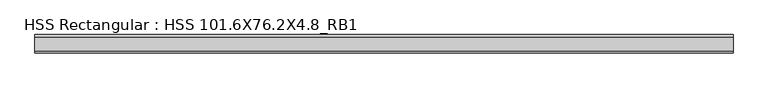
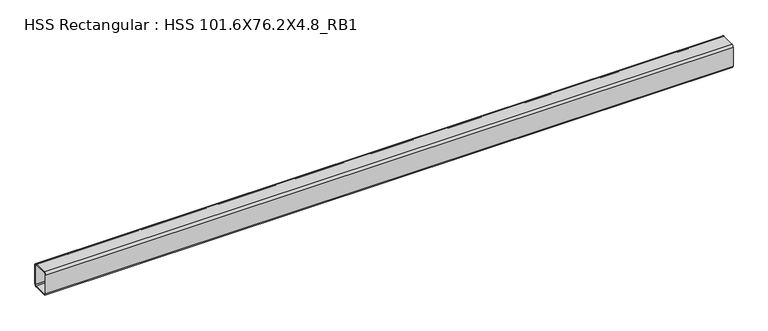
"""IFC4 building model written with IfcOpenShell, lengths in millimetres: beam geometry, HSS Rectangular : HSS 101.6X76.2X4.8_RB1."""

from ifc_helpers import new_model, si_unit, point, frame, frame_2d, origin, place, context, project, spatial, polyline, circle_curve, trimmed, segment, composite_curve, outline, extrude, source, transform, mapped, element, save


def hss_rectangular_hss_101_6x76_2x4_8_rb1_4e28bed8(model_context):
    return source(origin(), model_context, "Body", "SweptSolid", [
        extrude(outline(composite_curve([segment(polyline([(38.1, 41.275), (38.1, -41.275)]), True, "CONTINUOUS"), segment(trimmed(circle_curve(frame_2d((28.575, -41.275)), 9.525), [point((38.1, -41.275))], [point((28.575, -50.8))], False, "CARTESIAN"), True, "CONTINUOUS"), segment(polyline([(28.575, -50.8), (-28.575, -50.8)]), True, "CONTINUOUS"), segment(trimmed(circle_curve(frame_2d((-28.575, -41.275)), 9.525), [point((-28.575, -50.8))], [point((-38.1, -41.275))], False, "CARTESIAN"), True, "CONTINUOUS"), segment(polyline([(-38.1, -41.275), (-38.1, 41.275)]), True, "CONTINUOUS"), segment(trimmed(circle_curve(frame_2d((-28.575, 41.275)), 9.525), [point((-38.1, 41.275))], [point((-28.575, 50.8))], False, "CARTESIAN"), True, "CONTINUOUS"), segment(polyline([(-28.575, 50.8), (28.575, 50.8)]), True, "CONTINUOUS"), segment(trimmed(circle_curve(frame_2d((28.575, 41.275)), 9.525), [point((28.575, 50.8))], [point((38.1, 41.275))], False, "CARTESIAN"), True, "CONTINUOUS")], self_intersect=False), holes=[composite_curve([segment(trimmed(circle_curve(frame_2d((-28.575, 41.275)), 4.7625), [point((-28.575, 46.0375))], [point((-33.3375, 41.275))], True, "CARTESIAN"), True, "CONTINUOUS"), segment(polyline([(-33.3375, 41.275), (-33.3375, -41.275)]), True, "CONTINUOUS"), segment(trimmed(circle_curve(frame_2d((-28.575, -41.275)), 4.7625), [point((-33.3375, -41.275))], [point((-28.575, -46.0375))], True, "CARTESIAN"), True, "CONTINUOUS"), segment(polyline([(-28.575, -46.0375), (28.575, -46.0375)]), True, "CONTINUOUS"), segment(trimmed(circle_curve(frame_2d((28.575, -41.275)), 4.7625), [point((28.575, -46.0375))], [point((33.3375, -41.275))], True, "CARTESIAN"), True, "CONTINUOUS"), segment(polyline([(33.3375, -41.275), (33.3375, 41.275)]), True, "CONTINUOUS"), segment(trimmed(circle_curve(frame_2d((28.575, 41.275)), 4.7625), [point((33.3375, 41.275))], [point((28.575, 46.0375))], True, "CARTESIAN"), True, "CONTINUOUS"), segment(polyline([(28.575, 46.0375), (-28.575, 46.0375)]), True, "CONTINUOUS")], self_intersect=False)]), frame((-1474.1250006, 0.0, 0.0), z_axis=(1.0, 0.0, 0.0), x_axis=(0.0, 1.0, 0.0)), (0.0, 0.0, 1.0), 2884.7500012),
    ])


if __name__ == "__main__":
    model = new_model("IFC4")
    model_context = context("Model", 3, world=origin())
    ifc_project = project(units=[si_unit("LENGTHUNIT", "METRE", prefix="MILLI")], contexts=[model_context])
    site = spatial("IfcSite", under=ifc_project)
    building = spatial("IfcBuilding", under=site)
    placement = place(None, origin())
    hss_rectangular_hss_101_6x76_2x4_8_rb1_shape = hss_rectangular_hss_101_6x76_2x4_8_rb1_4e28bed8(model_context)
    element("IfcBeam", 1, ObjectType="HSS Rectangular : HSS 101.6X76.2X4.8_RB1", at=placement, inside=building, context=model_context, shape_type="MappedRepresentation", body=[
        mapped(hss_rectangular_hss_101_6x76_2x4_8_rb1_shape, transform((0.0, 0.0, 0.0), x_axis=(1.0, 0.0, 0.0), y_axis=(0.0, 1.0, 0.0), z_axis=(0.0, 0.0, 1.0))),
    ])
    save(model, "model.ifc")

# Revit data of these elements
# Type "HSS Rectangular : HSS 101.6X76.2X4.8_RB1"
#   Section Name Key = "HSS 4X3X3/16"
#   Assembly Code = "B10"
#   Width = 7.62 cm
#   Wall Nominal Thickness = 0.4763 cm
#   Wall Design Thickness = 0.442 cm
#   Torsional Moment of Inertia = 260.561 cm⁴
#   Torsional Modulus = 61.2876 cm³
#   Section Area = 14.4516 cm²
#   Plastic Modulus weak axis = 40.3122 cm³
#   Plastic Modulus strong axis = 49.1612 cm³
#   Perimeter = 0.881482 m²/m
#   Outer Fillet = 0.9525 cm
#   Nominal Weight = 12.1285 kgf/m
#   Moment of Inertia weak axis = 131.529 cm⁴
#   Moment of Inertia strong axis = 205.202 cm⁴
#   Inner Fillet = 0.4763 cm
#   Height = 10.16 cm
#   Elastic Modulus weak axis = 34.4128 cm³
#   Elastic Modulus strong axis = 40.476 cm³
#   Centroid Vertical = 5.08 cm
#   Centroid Horizontal = 3.81 cm
#   Length [instance default] = 1524 mm
#   Structural Material [instance default] = Steel ASTM A500, Grade B, Rectangular and Square
#   Principal Axes Angle = 0
# Element 1 (IfcBeam, "HSS Rectangular : HSS 101.6X76.2X4.8_RB1")
#   Structural Material = Steel ASTM A992
#   Materials on its faces: "Steel ASTM A992"
# Materials
#   "Steel ASTM A500, Grade B, Rectangular and Square": class "Metal", colour RGB 199 199 199, transparency 0, Description = "Carbon steel", Cost = 0
#   "Steel ASTM A992": class "Metal", colour RGB 199 199 199, transparency 0, Description = "Structural steel 50ksi", Cost = 0
